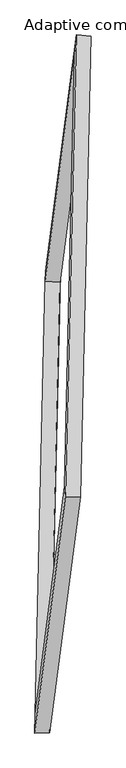
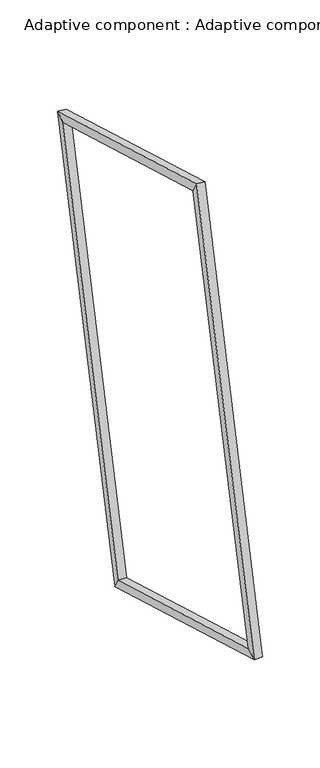
"""IFC4 building model written with IfcOpenShell, lengths in millimetres: proxy geometry, Adaptive component : Adaptive component."""

import ifcopenshell
import ifcopenshell.guid

model = None  # the IFC model being written
_history = None  # IfcOwnerHistory: only IFC2X3 demands one
_inside = {}  # id of a spatial element -> (the spatial element, [elements in it])
_under = {}  # id of a project, library or spatial element -> (it, [spatial elements below it])
_declared = {}  # id of a project -> (the project, [libraries it declares])
_typed = {}  # id of a type object -> (the type object, [elements of that type])
_made_of = {}  # id of a material, layer set ... -> (it, [elements and type objects made of it])


def new_model(schema):
    """Start an empty IFC model of exactly this schema.

    Asked for "IFC4X3", IfcOpenShell would pick the latest addendum, in which some entities
    have other attributes; the version numbers below select the first issue.
    IFC2X3 requires an IfcOwnerHistory on every rooted entity: one is made here for all.
    """
    global model, _history
    if schema == "IFC4X3":
        model = ifcopenshell.file(schema_version=(4, 3, 0, 0))
    else:
        model = ifcopenshell.file(schema=schema)
    _inside.clear()
    _under.clear()
    _declared.clear()
    _typed.clear()
    _made_of.clear()
    _history = None
    if model.schema == "IFC2X3":
        org = make("IfcOrganization", Name="unknown")
        user = make(
            "IfcPersonAndOrganization",
            ThePerson=make("IfcPerson", FamilyName="unknown"),
            TheOrganization=org,
        )
        app = make(
            "IfcApplication",
            ApplicationDeveloper=org,
            Version="unknown",
            ApplicationFullName="unknown",
            ApplicationIdentifier="unknown",
        )
        _history = make(
            "IfcOwnerHistory",
            OwningUser=user,
            OwningApplication=app,
            ChangeAction="ADDED",
            CreationDate=0,
        )
    return model


def make(cls, **values):
    """One entity of the class cls with the attributes given. An attribute that is None is left unset."""
    return model.create_entity(
        cls, **{name: value for name, value in values.items() if value is not None}
    )


def rooted(cls, **values):
    """An entity with a GlobalId (a new one), such as an element, a storey or a relation."""
    return make(cls, GlobalId=ifcopenshell.guid.new(), OwnerHistory=_history, **values)


def si_unit(unit_type, name, prefix=None):
    """IfcSIUnit, for example si_unit("LENGTHUNIT", "METRE", prefix="MILLI")."""
    return make("IfcSIUnit", UnitType=unit_type, Prefix=prefix, Name=name)


def assignment(units):
    """IfcUnitAssignment: the units of a project."""
    return None if units is None else make("IfcUnitAssignment", Units=units)


def point(xyz):
    """IfcCartesianPoint."""
    return None if xyz is None else make("IfcCartesianPoint", Coordinates=xyz)


def direction(xyz):
    """IfcDirection."""
    return None if xyz is None else make("IfcDirection", DirectionRatios=xyz)


def frame(location, z_axis=None, x_axis=None):
    """IfcAxis2Placement3D, a coordinate frame: its origin and axes. An axis left out is left unset."""
    return make(
        "IfcAxis2Placement3D",
        Location=point(location),
        Axis=direction(z_axis),
        RefDirection=direction(x_axis),
    )


def origin():
    """The frame at (0, 0, 0) with its axes left unset."""
    return frame((0.0, 0.0, 0.0))


def place(relative_to, where):
    """IfcLocalPlacement: puts the frame where relative to a parent placement (None: the world)."""
    return make(
        "IfcLocalPlacement", PlacementRelTo=relative_to, RelativePlacement=where
    )


def context(
    kind, dimensions, precision=None, world=None, true_north=None, identifier=None
):
    """IfcGeometricRepresentationContext, for example the 3D "Model" context."""
    return make(
        "IfcGeometricRepresentationContext",
        ContextIdentifier=identifier,
        ContextType=kind,
        CoordinateSpaceDimension=dimensions,
        Precision=precision,
        WorldCoordinateSystem=world,
        TrueNorth=true_north,
    )


def project(units=None, contexts=None):
    """IfcProject with its units and contexts."""
    return rooted(
        "IfcProject",
        Name="project",
        RepresentationContexts=contexts,
        UnitsInContext=assignment(units),
    )


def spatial(cls, under=None, at=None, **own):
    """A site, building, storey or space (cls), placed at a placement, below another one or the project."""
    s = rooted(cls, ObjectPlacement=at, **own)
    if under is not None:
        _under.setdefault(under.id(), (under, []))[1].append(s)
    return s


def faces_of(points, faces, orient=None, outer=None):
    """IfcFace entities. A face is a list of loops; a loop is a list of indices into points, from 0.

    orient and outer hold one flag for each loop. By default every Orientation is true, the
    first loop of a face is its IfcFaceOuterBound and the others are IfcFaceBound.
    """
    made = []
    for i, loops in enumerate(faces):
        bounds = []
        for j, loop in enumerate(loops):
            is_outer = j == 0 if outer is None else outer[i][j]
            bounds.append(
                make(
                    "IfcFaceOuterBound" if is_outer else "IfcFaceBound",
                    Bound=make("IfcPolyLoop", Polygon=[points[k] for k in loop]),
                    Orientation=True if orient is None else orient[i][j],
                )
            )
        made.append(make("IfcFace", Bounds=bounds))
    return made


def faceted_brep(points, faces, orient=None, outer=None, voids=None):
    """IfcFacetedBrep: a solid bounded by flat faces; with voids (closed shells), ...WithVoids."""
    shared = [point(p) for p in points]
    hull = make("IfcClosedShell", CfsFaces=faces_of(shared, faces, orient, outer))
    if voids is None:
        return make("IfcFacetedBrep", Outer=hull)
    return make(
        "IfcFacetedBrepWithVoids",
        Outer=hull,
        Voids=[
            make(cls, CfsFaces=faces_of(shared, fs, o, b)) for cls, fs, o, b in voids
        ],
    )


def shape(context_of_items, identifier, shape_type, items):
    """IfcShapeRepresentation: the items that make up one representation, for example the "Body"."""
    return make(
        "IfcShapeRepresentation",
        ContextOfItems=context_of_items,
        RepresentationIdentifier=identifier,
        RepresentationType=shape_type,
        Items=items,
    )


def source(mapping_origin, context_of_items, identifier, shape_type, items):
    """IfcRepresentationMap: a shape defined once, which mapped items show again and again."""
    return make(
        "IfcRepresentationMap",
        MappingOrigin=mapping_origin,
        MappedRepresentation=shape(context_of_items, identifier, shape_type, items),
    )


def transform(
    local_origin,
    x_axis=None,
    y_axis=None,
    z_axis=None,
    scale=None,
    scale2=None,
    scale3=None,
    uniform=True,
):
    """IfcCartesianTransformationOperator3D, or its non-uniform kind. x_axis, y_axis, z_axis: its Axis1, 2, 3."""
    if uniform:
        return make(
            "IfcCartesianTransformationOperator3D",
            Axis1=direction(x_axis),
            Axis2=direction(y_axis),
            LocalOrigin=point(local_origin),
            Scale=scale,
            Axis3=direction(z_axis),
        )
    return make(
        "IfcCartesianTransformationOperator3DnonUniform",
        Axis1=direction(x_axis),
        Axis2=direction(y_axis),
        LocalOrigin=point(local_origin),
        Scale=scale,
        Axis3=direction(z_axis),
        Scale2=scale2,
        Scale3=scale3,
    )


def mapped(mapping_source, mapping_target):
    """IfcMappedItem: shows the shape of a source again, moved by a transform."""
    return make(
        "IfcMappedItem", MappingSource=mapping_source, MappingTarget=mapping_target
    )


def made_of(thing, what):
    """Note that an element or type object is made of a material, layer set ...; save() writes the relation."""
    if what is not None:
        _made_of.setdefault(what.id(), (what, []))[1].append(thing)
    return thing


def element(
    cls,
    number,
    at=None,
    inside=None,
    cuts=None,
    type_object=None,
    material=None,
    context=None,
    identifier="Body",
    shape_type=None,
    held_by="IfcProductDefinitionShape",
    body=None,
    shapes=None,
    **own,
):
    """One element of the class cls, such as IfcWall. Its Tag is "e" and its number.

    at: its placement. inside: the storey or other place that contains it. cuts: it is an
    opening in that element (IfcRelVoidsElement). A single representation is given by context,
    identifier, shape_type and body (its items); several are given by shapes. held_by: the class
    of the entity that holds the representations. save() writes the other relations.
    """
    e = rooted(cls, Tag="e%d" % number, ObjectPlacement=at, **own)
    if body is not None:
        shapes = [shape(context, identifier, shape_type, body)]
    if shapes is not None:
        e.Representation = make(held_by, Representations=shapes)
    if inside is not None:
        _inside.setdefault(inside.id(), (inside, []))[1].append(e)
    if cuts is not None:
        rooted(
            "IfcRelVoidsElement", RelatingBuildingElement=cuts, RelatedOpeningElement=e
        )
    if type_object is not None:
        _typed.setdefault(type_object.id(), (type_object, []))[1].append(e)
    return made_of(e, material)


def aggregate(whole, parts):
    """IfcRelAggregates: a whole, such as a stair, and the parts it consists of."""
    return rooted("IfcRelAggregates", RelatingObject=whole, RelatedObjects=parts)


def save(model, path):
    """Write the relations noted so far, then the file.

    IfcRelAggregates (storeys below a building ...), IfcRelContainedInSpatialStructure (elements
    in a storey), IfcRelDefinesByType, IfcRelAssociatesMaterial and IfcRelDeclares: one each for
    every whole, place, type object, material and project.
    """
    for whole, parts in _under.values():
        aggregate(whole, parts)
    for where, things in _inside.values():
        rooted(
            "IfcRelContainedInSpatialStructure",
            RelatedElements=things,
            RelatingStructure=where,
        )
    for kind, things in _typed.values():
        rooted("IfcRelDefinesByType", RelatedObjects=things, RelatingType=kind)
    for what, things in _made_of.values():
        rooted("IfcRelAssociatesMaterial", RelatedObjects=things, RelatingMaterial=what)
    for by, libraries in _declared.values():
        rooted("IfcRelDeclares", RelatingContext=by, RelatedDefinitions=libraries)
    model.write(path)


def adaptive_component_adaptive_component_6b30b815(model_context):
    return source(origin(), model_context, "Body", "Brep", [
        faceted_brep([(63.4552574, 1018.6106139, 2666.4641461), (128.1277803, 1012.5944604, 2662.4706737), (83.7327773, -866.3413827, 3242.0437121), (18.9198182, -866.2689276, 3247.8705666), (70.5086918, 1099.6033884, 2709.2513219), (23.0422191, -909.3266927, 3328.9221399), (135.1812147, 1093.5872349, 2705.2578495), (87.8551781, -909.3991478, 3323.0952854), (-44.8795721, -1855.2186195, 26.3202279), (-109.9301986, -1856.9735468, 26.2046292), (-110.76814, -1938.1704916, -16.7683491), (-45.7175135, -1936.4155643, -16.6527504), (-0.4845691, 23.7172236, -553.2528104), (-65.3947594, 27.9059947, -555.2017912), (-63.3016672, 70.7595894, -636.4391671), (1.6085232, 66.5708184, -634.4901863)], [[[0, 1, 2, 3]], [[4, 0, 3, 5]], [[6, 4, 5, 7]], [[1, 6, 7, 2]], [[3, 2, 8, 9]], [[5, 3, 9, 10]], [[7, 5, 10, 11]], [[2, 7, 11, 8]], [[9, 8, 12, 13]], [[10, 9, 13, 14]], [[11, 10, 14, 15]], [[8, 11, 15, 12]], [[13, 12, 1, 0]], [[14, 13, 0, 4]], [[15, 14, 4, 6]], [[12, 15, 6, 1]]]),
    ])


if __name__ == "__main__":
    model = new_model("IFC4")
    model_context = context("Model", 3, world=origin())
    ifc_project = project(units=[si_unit("LENGTHUNIT", "METRE", prefix="MILLI")], contexts=[model_context])
    site = spatial("IfcSite", under=ifc_project)
    building = spatial("IfcBuilding", under=site)
    placement = place(None, origin())
    adaptive_component_adaptive_component_shape = adaptive_component_adaptive_component_6b30b815(model_context)
    element("IfcBuildingElementProxy", 1, Name="Adaptive component : Adaptive component", ObjectType="Adaptive component : Adaptive component", at=placement, inside=building, context=model_context, shape_type="MappedRepresentation", body=[
        mapped(adaptive_component_adaptive_component_shape, transform((0.0, 0.0, 0.0), x_axis=(1.0, 0.0, 0.0), y_axis=(0.0, 1.0, 0.0), z_axis=(0.0, 0.0, 1.0))),
    ])
    save(model, "model.ifc")

# Revit data of these elements
# Type "Adaptive component : Adaptive component"
#   r [instance default] = 2063.125 mm
#   2r [instance default] = 4126.251 mm
#   Number [instance default] = 5
#   Default Elevation = 0
# Element 1 (IfcBuildingElementProxy, "Adaptive component : Adaptive component")
#   r = 2040.833 mm
#   2r = 4081.666 mm
#   Number = 3
